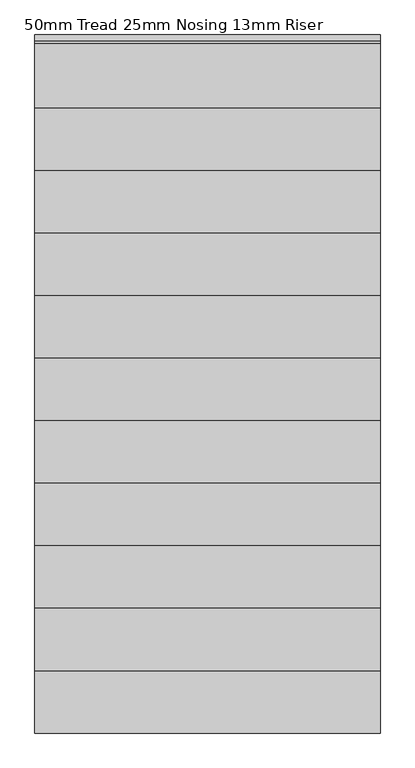
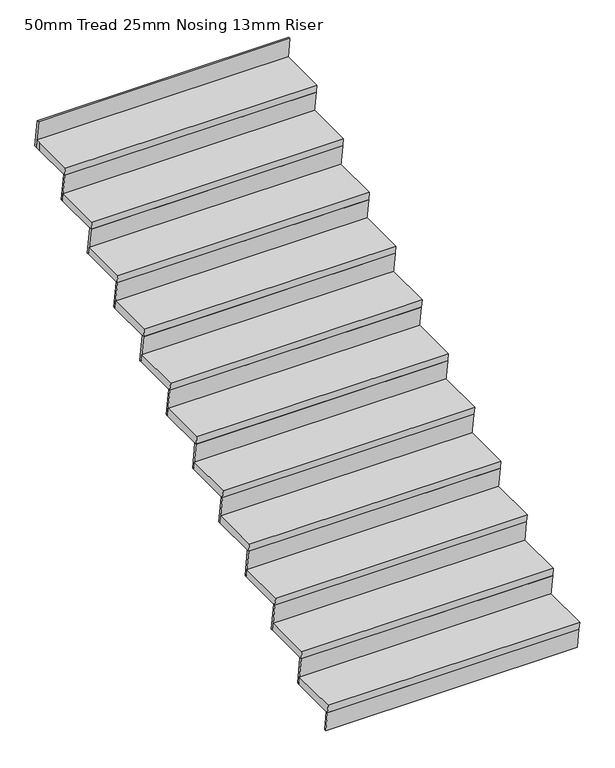
"""IFC4 building model written with IfcOpenShell, lengths in millimetres: stair flight geometry, 50mm Tread 25mm Nosing 13mm Riser."""

from ifc_helpers import new_model, si_unit, origin, place, context, project, spatial, faceted_brep, source, transform, mapped, element, save


def stair_flight_50mm_tread_25mm_nosing_13mm_riser_ea8afa7a(model_context):
    return source(origin(), model_context, "Body", "Brep", [
        faceted_brep([(-499.4393676, 4584.7509075, 9676.4705882), (-499.4393676, 4591.8342409, 9626.4705882), (-2019.4393676, 4591.8342409, 9626.4705882), (-2019.4393676, 4584.7509075, 9676.4705882), (-2019.4393676, 4284.7509075, 9676.4705882), (-499.4393676, 4284.7509075, 9676.4705882), (-499.4393676, 4291.8342409, 9626.4705882), (-2019.4393676, 4291.8342409, 9626.4705882)], [[[0, 1, 2, 3]], [[3, 4, 5, 0]], [[2, 1, 6, 7]], [[4, 3, 2, 7]], [[0, 5, 6, 1]], [[5, 4, 7, 6]]]),
        faceted_brep([(-499.4393676, 4291.8342409, 9626.4705882), (-499.4393676, 4309.7509075, 9500.0), (-499.4393676, 4322.3757185, 9500.0), (-499.4393676, 4304.4590518, 9626.4705882), (-2019.4393676, 4291.8342409, 9626.4705882), (-2019.4393676, 4304.4590518, 9626.4705882), (-2019.4393676, 4322.3757185, 9500.0), (-2019.4393676, 4309.7509075, 9500.0)], [[[0, 1, 2, 3]], [[4, 5, 6, 7]], [[1, 0, 4, 7]], [[2, 1, 7, 6]], [[3, 2, 6, 5]], [[0, 3, 5, 4]]]),
        faceted_brep([(-499.4393676, 4566.8342409, 9802.9411765), (-499.4393676, 4591.8342409, 9626.4705882), (-499.4393676, 4604.4590518, 9626.4705882), (-499.4393676, 4579.4590518, 9802.9411765), (-2019.4393676, 4566.8342409, 9802.9411765), (-2019.4393676, 4579.4590518, 9802.9411765), (-2019.4393676, 4604.4590518, 9626.4705882), (-2019.4393676, 4591.8342409, 9626.4705882)], [[[0, 1, 2, 3]], [[4, 5, 6, 7]], [[1, 0, 4, 7]], [[2, 1, 7, 6]], [[3, 2, 6, 5]], [[0, 3, 5, 4]]]),
        faceted_brep([(-2019.4393676, 4859.7509075, 9852.9411765), (-2019.4393676, 4559.7509075, 9852.9411765), (-499.4393676, 4559.7509075, 9852.9411765), (-499.4393676, 4859.7509075, 9852.9411765), (-2019.4393676, 4866.8342409, 9802.9411765), (-499.4393676, 4866.8342409, 9802.9411765), (-499.4393676, 4566.8342409, 9802.9411765), (-2019.4393676, 4566.8342409, 9802.9411765)], [[[0, 1, 2, 3]], [[4, 5, 6, 7]], [[1, 0, 4, 7]], [[3, 2, 6, 5]], [[3, 5, 4, 0]], [[2, 1, 7, 6]]]),
        faceted_brep([(-499.4393676, 4841.8342409, 9979.4117647), (-499.4393676, 4866.8342409, 9802.9411765), (-499.4393676, 4879.4590518, 9802.9411765), (-499.4393676, 4854.4590518, 9979.4117647), (-2019.4393676, 4841.8342409, 9979.4117647), (-2019.4393676, 4854.4590518, 9979.4117647), (-2019.4393676, 4879.4590518, 9802.9411765), (-2019.4393676, 4866.8342409, 9802.9411765)], [[[0, 1, 2, 3]], [[4, 5, 6, 7]], [[1, 0, 4, 7]], [[2, 1, 7, 6]], [[3, 2, 6, 5]], [[0, 3, 5, 4]]]),
        faceted_brep([(-2019.4393676, 5134.7509075, 10029.4117647), (-2019.4393676, 4834.7509075, 10029.4117647), (-499.4393676, 4834.7509075, 10029.4117647), (-499.4393676, 5134.7509075, 10029.4117647), (-2019.4393676, 5141.8342409, 9979.4117647), (-499.4393676, 5141.8342409, 9979.4117647), (-499.4393676, 4841.8342409, 9979.4117647), (-2019.4393676, 4841.8342409, 9979.4117647)], [[[0, 1, 2, 3]], [[4, 5, 6, 7]], [[1, 0, 4, 7]], [[3, 2, 6, 5]], [[3, 5, 4, 0]], [[2, 1, 7, 6]]]),
        faceted_brep([(-499.4393676, 5116.8342409, 10155.8823529), (-499.4393676, 5141.8342409, 9979.4117647), (-499.4393676, 5154.4590518, 9979.4117647), (-499.4393676, 5129.4590518, 10155.8823529), (-2019.4393676, 5116.8342409, 10155.8823529), (-2019.4393676, 5129.4590518, 10155.8823529), (-2019.4393676, 5154.4590518, 9979.4117647), (-2019.4393676, 5141.8342409, 9979.4117647)], [[[0, 1, 2, 3]], [[4, 5, 6, 7]], [[1, 0, 4, 7]], [[2, 1, 7, 6]], [[3, 2, 6, 5]], [[0, 3, 5, 4]]]),
        faceted_brep([(-2019.4393676, 5409.7509075, 10205.8823529), (-2019.4393676, 5109.7509075, 10205.8823529), (-499.4393676, 5109.7509075, 10205.8823529), (-499.4393676, 5409.7509075, 10205.8823529), (-2019.4393676, 5416.8342409, 10155.8823529), (-499.4393676, 5416.8342409, 10155.8823529), (-499.4393676, 5116.8342409, 10155.8823529), (-2019.4393676, 5116.8342409, 10155.8823529)], [[[0, 1, 2, 3]], [[4, 5, 6, 7]], [[1, 0, 4, 7]], [[3, 2, 6, 5]], [[3, 5, 4, 0]], [[2, 1, 7, 6]]]),
        faceted_brep([(-499.4393676, 5391.8342409, 10332.3529412), (-499.4393676, 5416.8342409, 10155.8823529), (-499.4393676, 5429.4590518, 10155.8823529), (-499.4393676, 5404.4590518, 10332.3529412), (-2019.4393676, 5391.8342409, 10332.3529412), (-2019.4393676, 5404.4590518, 10332.3529412), (-2019.4393676, 5429.4590518, 10155.8823529), (-2019.4393676, 5416.8342409, 10155.8823529)], [[[0, 1, 2, 3]], [[4, 5, 6, 7]], [[1, 0, 4, 7]], [[2, 1, 7, 6]], [[3, 2, 6, 5]], [[0, 3, 5, 4]]]),
        faceted_brep([(-2019.4393676, 5684.7509075, 10382.3529412), (-2019.4393676, 5384.7509075, 10382.3529412), (-499.4393676, 5384.7509075, 10382.3529412), (-499.4393676, 5684.7509075, 10382.3529412), (-2019.4393676, 5691.8342409, 10332.3529412), (-499.4393676, 5691.8342409, 10332.3529412), (-499.4393676, 5391.8342409, 10332.3529412), (-2019.4393676, 5391.8342409, 10332.3529412)], [[[0, 1, 2, 3]], [[4, 5, 6, 7]], [[1, 0, 4, 7]], [[3, 2, 6, 5]], [[3, 5, 4, 0]], [[2, 1, 7, 6]]]),
        faceted_brep([(-499.4393676, 5666.8342409, 10508.8235294), (-499.4393676, 5691.8342409, 10332.3529412), (-499.4393676, 5704.4590518, 10332.3529412), (-499.4393676, 5679.4590518, 10508.8235294), (-2019.4393676, 5666.8342409, 10508.8235294), (-2019.4393676, 5679.4590518, 10508.8235294), (-2019.4393676, 5704.4590518, 10332.3529412), (-2019.4393676, 5691.8342409, 10332.3529412)], [[[0, 1, 2, 3]], [[4, 5, 6, 7]], [[1, 0, 4, 7]], [[2, 1, 7, 6]], [[3, 2, 6, 5]], [[0, 3, 5, 4]]]),
        faceted_brep([(-2019.4393676, 5959.7509075, 10558.8235294), (-2019.4393676, 5659.7509075, 10558.8235294), (-499.4393676, 5659.7509075, 10558.8235294), (-499.4393676, 5959.7509075, 10558.8235294), (-2019.4393676, 5966.8342409, 10508.8235294), (-499.4393676, 5966.8342409, 10508.8235294), (-499.4393676, 5666.8342409, 10508.8235294), (-2019.4393676, 5666.8342409, 10508.8235294)], [[[0, 1, 2, 3]], [[4, 5, 6, 7]], [[1, 0, 4, 7]], [[3, 2, 6, 5]], [[3, 5, 4, 0]], [[2, 1, 7, 6]]]),
        faceted_brep([(-499.4393676, 5941.8342409, 10685.2941176), (-499.4393676, 5966.8342409, 10508.8235294), (-499.4393676, 5979.4590518, 10508.8235294), (-499.4393676, 5954.4590518, 10685.2941176), (-2019.4393676, 5941.8342409, 10685.2941176), (-2019.4393676, 5954.4590518, 10685.2941176), (-2019.4393676, 5979.4590518, 10508.8235294), (-2019.4393676, 5966.8342409, 10508.8235294)], [[[0, 1, 2, 3]], [[4, 5, 6, 7]], [[1, 0, 4, 7]], [[2, 1, 7, 6]], [[3, 2, 6, 5]], [[0, 3, 5, 4]]]),
        faceted_brep([(-2019.4393676, 6234.7509075, 10735.2941176), (-2019.4393676, 5934.7509075, 10735.2941176), (-499.4393676, 5934.7509075, 10735.2941176), (-499.4393676, 6234.7509075, 10735.2941176), (-2019.4393676, 6241.8342409, 10685.2941176), (-499.4393676, 6241.8342409, 10685.2941176), (-499.4393676, 5941.8342409, 10685.2941176), (-2019.4393676, 5941.8342409, 10685.2941176)], [[[0, 1, 2, 3]], [[4, 5, 6, 7]], [[1, 0, 4, 7]], [[3, 2, 6, 5]], [[3, 5, 4, 0]], [[2, 1, 7, 6]]]),
        faceted_brep([(-499.4393676, 6216.8342409, 10861.7647059), (-499.4393676, 6241.8342409, 10685.2941176), (-499.4393676, 6254.4590518, 10685.2941176), (-499.4393676, 6229.4590518, 10861.7647059), (-2019.4393676, 6216.8342409, 10861.7647059), (-2019.4393676, 6229.4590518, 10861.7647059), (-2019.4393676, 6254.4590518, 10685.2941176), (-2019.4393676, 6241.8342409, 10685.2941176)], [[[0, 1, 2, 3]], [[4, 5, 6, 7]], [[1, 0, 4, 7]], [[2, 1, 7, 6]], [[3, 2, 6, 5]], [[0, 3, 5, 4]]]),
        faceted_brep([(-2019.4393676, 6509.7509075, 10911.7647059), (-2019.4393676, 6209.7509075, 10911.7647059), (-499.4393676, 6209.7509075, 10911.7647059), (-499.4393676, 6509.7509075, 10911.7647059), (-2019.4393676, 6516.8342409, 10861.7647059), (-499.4393676, 6516.8342409, 10861.7647059), (-499.4393676, 6216.8342409, 10861.7647059), (-2019.4393676, 6216.8342409, 10861.7647059)], [[[0, 1, 2, 3]], [[4, 5, 6, 7]], [[1, 0, 4, 7]], [[3, 2, 6, 5]], [[3, 5, 4, 0]], [[2, 1, 7, 6]]]),
        faceted_brep([(-499.4393676, 6491.8342409, 11038.2352941), (-499.4393676, 6516.8342409, 10861.7647059), (-499.4393676, 6529.4590518, 10861.7647059), (-499.4393676, 6504.4590518, 11038.2352941), (-2019.4393676, 6491.8342409, 11038.2352941), (-2019.4393676, 6504.4590518, 11038.2352941), (-2019.4393676, 6529.4590518, 10861.7647059), (-2019.4393676, 6516.8342409, 10861.7647059)], [[[0, 1, 2, 3]], [[4, 5, 6, 7]], [[1, 0, 4, 7]], [[2, 1, 7, 6]], [[3, 2, 6, 5]], [[0, 3, 5, 4]]]),
        faceted_brep([(-2019.4393676, 6784.7509075, 11088.2352941), (-2019.4393676, 6484.7509075, 11088.2352941), (-499.4393676, 6484.7509075, 11088.2352941), (-499.4393676, 6784.7509075, 11088.2352941), (-2019.4393676, 6791.8342409, 11038.2352941), (-499.4393676, 6791.8342409, 11038.2352941), (-499.4393676, 6491.8342409, 11038.2352941), (-2019.4393676, 6491.8342409, 11038.2352941)], [[[0, 1, 2, 3]], [[4, 5, 6, 7]], [[1, 0, 4, 7]], [[3, 2, 6, 5]], [[3, 5, 4, 0]], [[2, 1, 7, 6]]]),
        faceted_brep([(-499.4393676, 6766.8342409, 11214.7058824), (-499.4393676, 6791.8342409, 11038.2352941), (-499.4393676, 6804.4590518, 11038.2352941), (-499.4393676, 6779.4590518, 11214.7058824), (-2019.4393676, 6766.8342409, 11214.7058824), (-2019.4393676, 6779.4590518, 11214.7058824), (-2019.4393676, 6804.4590518, 11038.2352941), (-2019.4393676, 6791.8342409, 11038.2352941)], [[[0, 1, 2, 3]], [[4, 5, 6, 7]], [[1, 0, 4, 7]], [[2, 1, 7, 6]], [[3, 2, 6, 5]], [[0, 3, 5, 4]]]),
        faceted_brep([(-2019.4393676, 7059.7509075, 11264.7058824), (-2019.4393676, 6759.7509075, 11264.7058824), (-499.4393676, 6759.7509075, 11264.7058824), (-499.4393676, 7059.7509075, 11264.7058824), (-2019.4393676, 7066.8342409, 11214.7058824), (-499.4393676, 7066.8342409, 11214.7058824), (-499.4393676, 6766.8342409, 11214.7058824), (-2019.4393676, 6766.8342409, 11214.7058824)], [[[0, 1, 2, 3]], [[4, 5, 6, 7]], [[1, 0, 4, 7]], [[3, 2, 6, 5]], [[3, 5, 4, 0]], [[2, 1, 7, 6]]]),
        faceted_brep([(-499.4393676, 7316.8342409, 11567.6470588), (-499.4393676, 7341.8342409, 11391.1764706), (-499.4393676, 7354.4590518, 11391.1764706), (-499.4393676, 7329.4590518, 11567.6470588), (-2019.4393676, 7316.8342409, 11567.6470588), (-2019.4393676, 7329.4590518, 11567.6470588), (-2019.4393676, 7354.4590518, 11391.1764706), (-2019.4393676, 7341.8342409, 11391.1764706)], [[[0, 1, 2, 3]], [[4, 5, 6, 7]], [[1, 0, 4, 7]], [[2, 1, 7, 6]], [[3, 2, 6, 5]], [[0, 3, 5, 4]]]),
        faceted_brep([(-499.4393676, 7041.8342409, 11391.1764706), (-499.4393676, 7066.8342409, 11214.7058824), (-499.4393676, 7079.4590518, 11214.7058824), (-499.4393676, 7054.4590518, 11391.1764706), (-2019.4393676, 7041.8342409, 11391.1764706), (-2019.4393676, 7054.4590518, 11391.1764706), (-2019.4393676, 7079.4590518, 11214.7058824), (-2019.4393676, 7066.8342409, 11214.7058824)], [[[0, 1, 2, 3]], [[4, 5, 6, 7]], [[1, 0, 4, 7]], [[2, 1, 7, 6]], [[3, 2, 6, 5]], [[0, 3, 5, 4]]]),
        faceted_brep([(-2019.4393676, 7334.7509075, 11441.1764706), (-2019.4393676, 7309.7509075, 11441.1764706), (-2019.4393676, 7034.7509075, 11441.1764706), (-499.4393676, 7034.7509075, 11441.1764706), (-499.4393676, 7334.7509075, 11441.1764706), (-2019.4393676, 7341.8342409, 11391.1764706), (-499.4393676, 7341.8342409, 11391.1764706), (-499.4393676, 7041.8342409, 11391.1764706), (-2019.4393676, 7041.8342409, 11391.1764706), (-2019.4393676, 7309.7509075, 11391.1764706)], [[[0, 1, 2, 3, 4]], [[5, 6, 7, 8, 9]], [[1, 0, 5, 9]], [[2, 1, 9, 8]], [[4, 3, 7, 6]], [[4, 6, 5, 0]], [[3, 2, 8, 7]]]),
    ])


if __name__ == "__main__":
    model = new_model("IFC4")
    model_context = context("Model", 3, world=origin())
    ifc_project = project(units=[si_unit("LENGTHUNIT", "METRE", prefix="MILLI")], contexts=[model_context])
    site = spatial("IfcSite", under=ifc_project)
    building = spatial("IfcBuilding", under=site)
    placement = place(None, origin())
    stair_flight_50mm_tread_25mm_nosing_13mm_riser_shape = stair_flight_50mm_tread_25mm_nosing_13mm_riser_ea8afa7a(model_context)
    element("IfcStairFlight", 1, ObjectType="50mm Tread 25mm Nosing 13mm Riser", at=placement, inside=building, context=model_context, shape_type="MappedRepresentation", body=[
        mapped(stair_flight_50mm_tread_25mm_nosing_13mm_riser_shape, transform((0.0, 0.0, 0.0), x_axis=(1.0, 0.0, 0.0), y_axis=(0.0, 1.0, 0.0), z_axis=(0.0, 0.0, 1.0))),
    ])
    save(model, "model.ifc")
